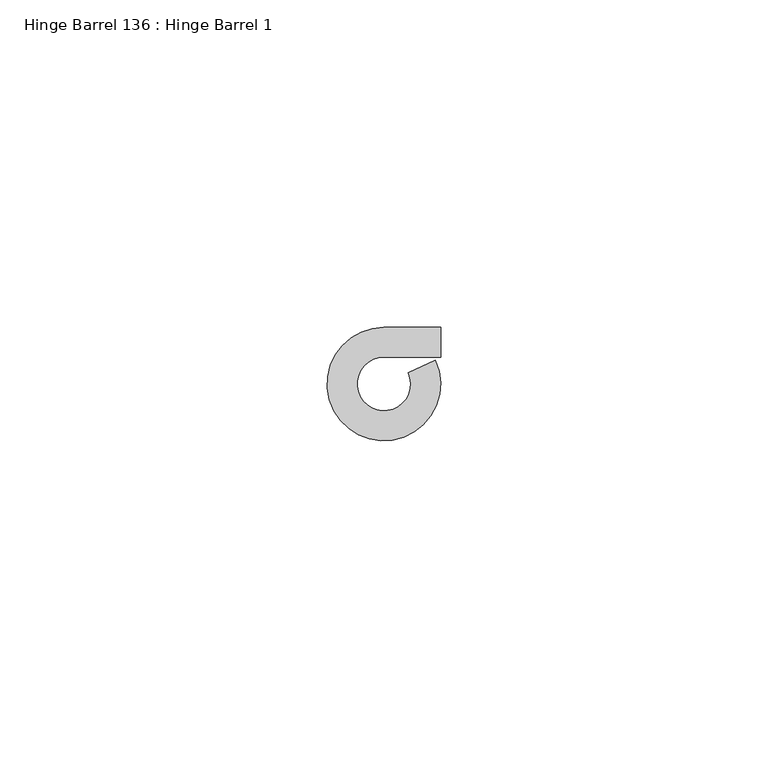
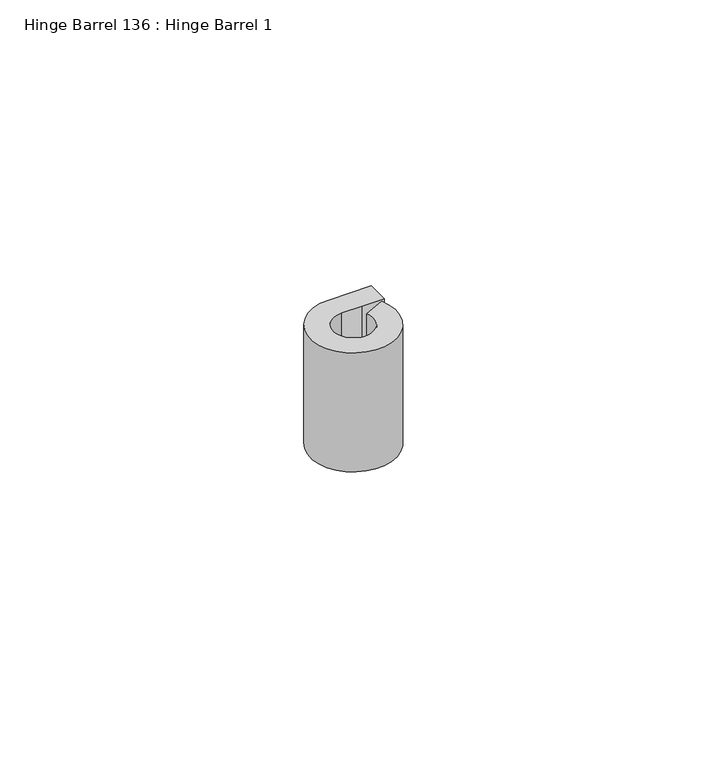
"""IFC4 building model written with IfcOpenShell, lengths in millimetres: proxy geometry, Hinge Barrel 136 : Hinge Barrel 1."""

from ifc_helpers import new_model, si_unit, point, frame, frame_2d, origin, place, context, project, spatial, polyline, circle_curve, trimmed, segment, composite_curve, outline, extrude, source, transform, mapped, element, save


def hinge_barrel_136_hinge_barrel_1_8ace309c(model_context):
    return source(origin(), model_context, "Body", "SweptSolid", [
        extrude(outline(composite_curve([segment(polyline([(587323.2214739, -536306.2758841), (587319.1320739, -536306.2758841)]), True, "CONTINUOUS"), segment(trimmed(circle_curve(frame_2d((587319.1320739, -536310.3652841)), 4.0894), [point((587319.1320739, -536306.2758841))], [point((587322.8436736, -536308.6485371))], True, "CARTESIAN"), True, "CONTINUOUS"), segment(polyline([(587322.8436736, -536308.6485371), (587326.986084, -536306.7325249)]), True, "CONTINUOUS"), segment(trimmed(circle_curve(frame_2d((587319.1320739, -536310.3652841)), 8.6534625), [point((587326.986084, -536306.7325249))], [point((587319.1320739, -536301.7118216))], False, "CARTESIAN"), True, "CONTINUOUS"), segment(polyline([(587319.1320739, -536301.7118216), (587327.7934739, -536301.7118216), (587327.7934739, -536306.2758841), (587323.2214739, -536306.2758841)]), True, "CONTINUOUS")], self_intersect=False)), frame((0.0, 0.0, 2038.35), z_axis=(0.0, 0.0, 1.0), x_axis=(1.0, 0.0, 0.0)), (0.0, 0.0, 1.0), 25.4),
    ])


if __name__ == "__main__":
    model = new_model("IFC4")
    model_context = context("Model", 3, world=origin())
    ifc_project = project(units=[si_unit("LENGTHUNIT", "METRE", prefix="MILLI")], contexts=[model_context])
    site = spatial("IfcSite", under=ifc_project)
    building = spatial("IfcBuilding", under=site)
    placement = place(None, origin())
    hinge_barrel_136_hinge_barrel_1_shape = hinge_barrel_136_hinge_barrel_1_8ace309c(model_context)
    element("IfcBuildingElementProxy", 1, Name="Hinge Barrel 136 : Hinge Barrel 1", ObjectType="Hinge Barrel 136 : Hinge Barrel 1", at=placement, inside=building, context=model_context, shape_type="MappedRepresentation", body=[
        mapped(hinge_barrel_136_hinge_barrel_1_shape, transform((0.0, 0.0, 0.0), x_axis=(1.0, 0.0, 0.0), y_axis=(0.0, 1.0, 0.0), z_axis=(0.0, 0.0, 1.0))),
    ])
    save(model, "model.ifc")

# Revit data of these elements
# Element 1 (IfcBuildingElementProxy, "Hinge Barrel 136 : Hinge Barrel 1")
#   Materials on its faces: "6\"X6\" WELD-ON STL BUTT HINGE"
# Materials
#   "6\"X6\" WELD-ON STL BUTT HINGE": class "Metal", colour RGB 189 187 185, transparency 0, Description = "Carbon steel", Cost = 0
